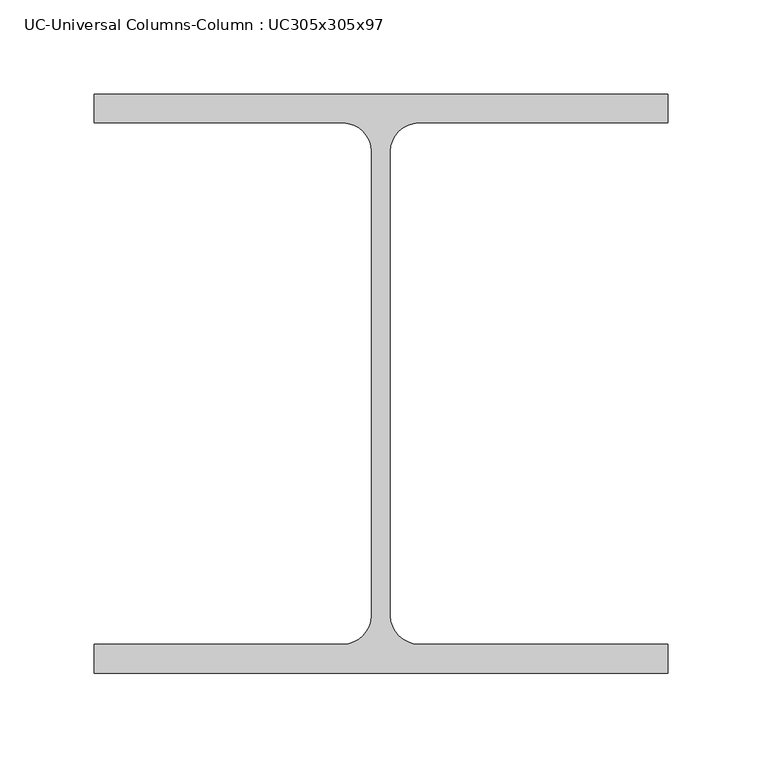
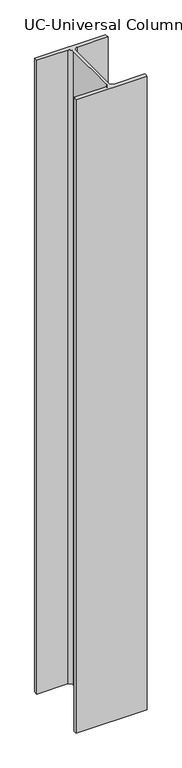
"""IFC4 building model written with IfcOpenShell, lengths in millimetres: column geometry, UC-Universal Columns-Column : UC305x305x97."""

from ifc_helpers import new_model, si_unit, point, frame, frame_2d, origin, place, context, project, spatial, polyline, circle_curve, trimmed, segment, composite_curve, outline, extrude, source, transform, mapped, element, save


def uc_universal_columns_column_uc305x305x97_1fa90765(model_context):
    return source(origin(), model_context, "Body", "SweptSolid", [
        extrude(outline(composite_curve([segment(polyline([(152.65, 153.95), (152.65, 138.55), (20.15, 138.55)]), True, "CONTINUOUS"), segment(trimmed(circle_curve(frame_2d((20.15, 123.35)), 15.2), [point((20.15, 138.55))], [point((4.95, 123.35))], True, "CARTESIAN"), True, "CONTINUOUS"), segment(polyline([(4.95, 123.35), (4.95, -123.35)]), True, "CONTINUOUS"), segment(trimmed(circle_curve(frame_2d((20.15, -123.35)), 15.2), [point((4.95, -123.35))], [point((20.15, -138.55))], True, "CARTESIAN"), True, "CONTINUOUS"), segment(polyline([(20.15, -138.55), (152.65, -138.55), (152.65, -153.95), (-152.65, -153.95), (-152.65, -138.55), (-20.15, -138.55)]), True, "CONTINUOUS"), segment(trimmed(circle_curve(frame_2d((-20.15, -123.35)), 15.2), [point((-20.15, -138.55))], [point((-4.95, -123.35))], True, "CARTESIAN"), True, "CONTINUOUS"), segment(polyline([(-4.95, -123.35), (-4.95, 123.35)]), True, "CONTINUOUS"), segment(trimmed(circle_curve(frame_2d((-20.15, 123.35)), 15.2), [point((-4.95, 123.35))], [point((-20.15, 138.55))], True, "CARTESIAN"), True, "CONTINUOUS"), segment(polyline([(-20.15, 138.55), (-152.65, 138.55), (-152.65, 153.95), (152.65, 153.95)]), True, "CONTINUOUS")], self_intersect=False)), frame((0.0, 0.0, 450.0), z_axis=(0.0, 0.0, 1.0), x_axis=(1.0, 0.0, 0.0)), (0.0, 0.0, 1.0), 2877.4),
    ])


if __name__ == "__main__":
    model = new_model("IFC4")
    model_context = context("Model", 3, world=origin())
    ifc_project = project(units=[si_unit("LENGTHUNIT", "METRE", prefix="MILLI")], contexts=[model_context])
    site = spatial("IfcSite", under=ifc_project)
    building = spatial("IfcBuilding", under=site)
    placement = place(None, origin())
    uc_universal_columns_column_uc305x305x97_shape = uc_universal_columns_column_uc305x305x97_1fa90765(model_context)
    element("IfcColumn", 1, ObjectType="UC-Universal Columns-Column : UC305x305x97", at=placement, inside=building, context=model_context, shape_type="MappedRepresentation", body=[
        mapped(uc_universal_columns_column_uc305x305x97_shape, transform((0.0, 0.0, 0.0), x_axis=(1.0, 0.0, 0.0), y_axis=(0.0, 1.0, 0.0), z_axis=(0.0, 0.0, 1.0))),
    ])
    save(model, "model.ifc")

# Revit data of these elements
# Type "UC-Universal Columns-Column : UC305x305x97"
#   Section Name Key = "UC305x305x97"
#   Width = 30.53 cm
#   Web Thickness = 0.99 cm
#   Web Fillet = 1.52 cm
#   Warping Constant = 1560000.0 cm⁶
#   Torsional Moment of Inertia = 91.20 cm⁴
#   Section Area = 123.0 cm²
#   Plastic Modulus weak axis = 726.0 cm³
#   Plastic Modulus strong axis = 1592.0 cm³
#   Nominal Weight = 96.8996 kgf/m
#   Moment of Inertia weak axis = 7308.00 cm⁴
#   Moment of Inertia strong axis = 22249.00 cm⁴
#   Height = 30.79 cm
#   Flange Thickness = 1.54 cm
#   Elastic Modulus weak axis = 479.0 cm³
#   Elastic Modulus strong axis = 1445.0 cm³
#   Centroid Vertical = 15.395 cm
#   Centroid Horizontal = 15.265 cm
#   Bolt Spacing = 14.0 cm
#   Structural Material [instance default] = Metal - Steel 43-275
#   Type Comments = ""
#   Assembly Code = ""
# Element 1 (IfcColumn, "UC-Universal Columns-Column : UC305x305x97")
#   Materials on its faces: "Metal - Steel 43-275"
# Materials
#   "Metal - Steel 43-275": class "Metal", colour RGB 247 247 247, transparency 0, Cost = 0
